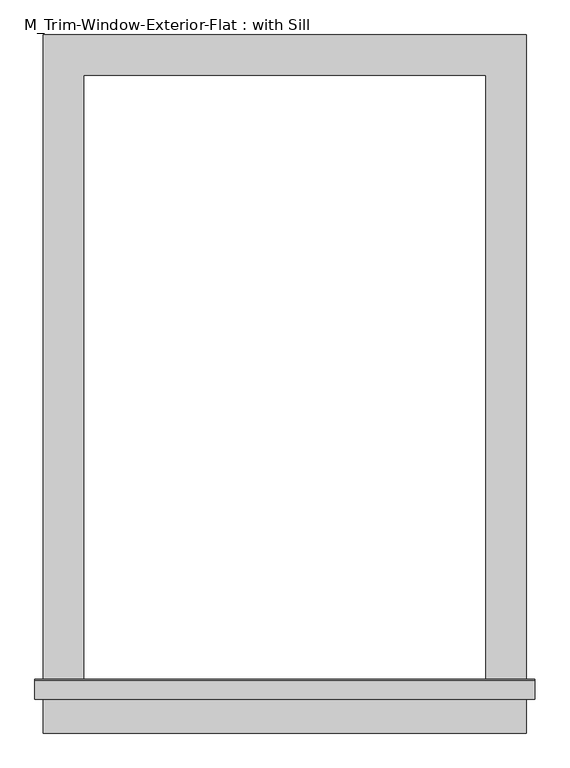
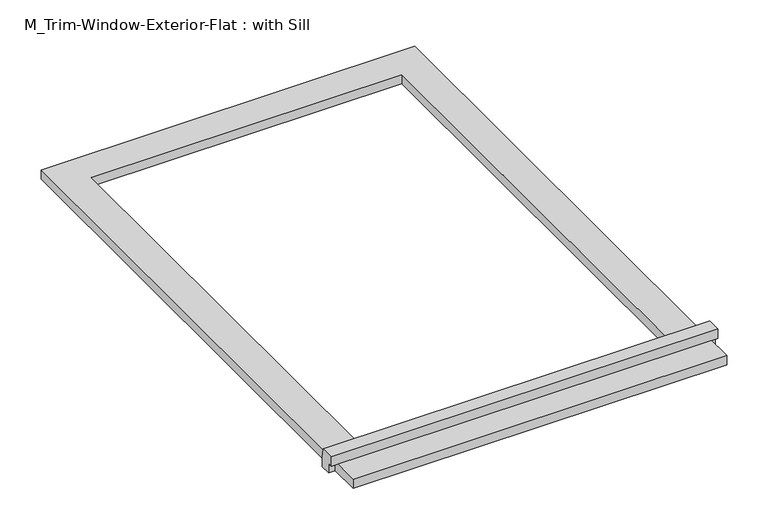
"""IFC4 building model written with IfcOpenShell, lengths in millimetres: proxy geometry, M_Trim-Window-Exterior-Flat : with Sill."""

from ifc_helpers import new_model, si_unit, frame, origin, origin_with_axes, place, context, project, spatial, polyline, outline, extrude, source, transform, mapped, element, save


def m_trim_window_exterior_flat_with_sill_a9fd4a74(model_context):
    return source(origin(), model_context, "Body", "SweptSolid", [
        extrude(outline(polyline([(360.0, -920.4323709), (360.0, -980.4323709), (-360.0, -980.4323709), (-360.0, -920.4323709), (360.0, -920.4323709)])), origin_with_axes(), (0.0, 0.0, 1.0), 19.05),
        extrude(outline(polyline([(-930.0, 38.1), (-902.4580645, 38.1), (-900.0, 19.05), (-900.0, 0.0), (-920.4323709, 0.0), (-920.4323709, 19.05), (-930.0, 19.05), (-930.0, 38.1)])), frame((-372.7, 0.0, 0.0), z_axis=(1.0, 0.0, 0.0), x_axis=(0.0, 1.0, 0.0)), (0.0, 0.0, 1.0), 745.4),
        extrude(outline(polyline([(-360.0, 60.0), (360.0, 60.0), (360.0, -900.0), (300.0, -900.0), (300.0, 0.0), (-300.0, 0.0), (-300.0, -900.0), (-360.0, -900.0), (-360.0, 60.0)])), origin_with_axes(), (0.0, 0.0, 1.0), 19.05),
    ])


if __name__ == "__main__":
    model = new_model("IFC4")
    model_context = context("Model", 3, world=origin())
    ifc_project = project(units=[si_unit("LENGTHUNIT", "METRE", prefix="MILLI")], contexts=[model_context])
    site = spatial("IfcSite", under=ifc_project)
    building = spatial("IfcBuilding", under=site)
    placement = place(None, origin())
    m_trim_window_exterior_flat_with_sill_shape = m_trim_window_exterior_flat_with_sill_a9fd4a74(model_context)
    element("IfcBuildingElementProxy", 1, Name="M_Trim-Window-Exterior-Flat : with Sill", ObjectType="M_Trim-Window-Exterior-Flat : with Sill", at=placement, inside=building, context=model_context, shape_type="MappedRepresentation", body=[
        mapped(m_trim_window_exterior_flat_with_sill_shape, transform((0.0, 0.0, 0.0), x_axis=(1.0, 0.0, 0.0), y_axis=(0.0, 1.0, 0.0), z_axis=(0.0, 0.0, 1.0))),
    ])
    save(model, "model.ifc")

# Revit data of these elements
# Type "M_Trim-Window-Exterior-Flat : with Sill"
#   Trim Width = 6 cm
#   Trim Thickness_Picture Frame = 3 cm
#   Trim Thickness_with Sill = 1.905 cm
#   Sill Thickness = 3 cm
#   Opening Width [instance default] = 60 cm
#   Opening Height [instance default] = 90 cm
#   Default Elevation = 120 cm
#   Sill = yes
#   Picture Frame = no
#   Trim Material [instance default] = none
# Element 1 (IfcBuildingElementProxy, "M_Trim-Window-Exterior-Flat : with Sill")
#   Trim Material = Clad - White
#   Materials on its faces: "Clad - White"
# Materials
#   "Clad - White": class "Wood", colour RGB 245 245 243, transparency 0, Cost = 0
